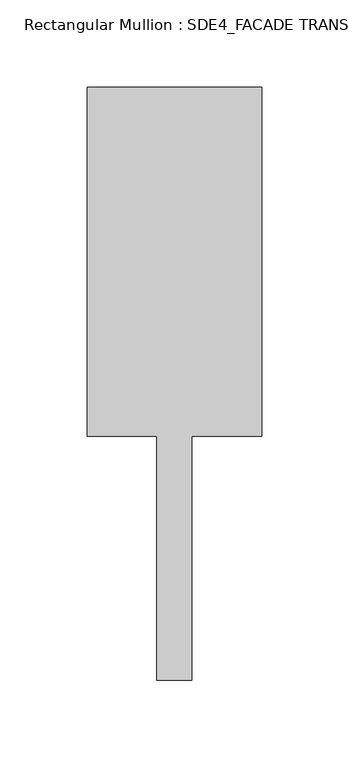
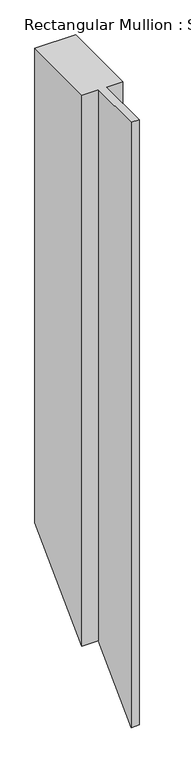
"""IFC4 building model written with IfcOpenShell, lengths in millimetres: member geometry, Rectangular Mullion : SDE4_FACADE TRANSOM TYPE 1."""

from ifc_helpers import new_model, si_unit, origin, place, context, project, spatial, faceted_brep, source, transform, mapped, element, save


def rectangular_mullion_sde4_facade_transom_type_1_05d00b60(model_context):
    return source(origin(), model_context, "Body", "Brep", [
        faceted_brep([(50.0, 132.5, 0.0), (-50.0, 132.5, 0.0), (-50.0, -67.5, 0.0), (-10.0, -67.5, 0.0), (-10.0, -207.5, 0.0), (10.0, -207.5, 0.0), (10.0, -67.5, 0.0), (50.0, -67.5, 0.0), (50.0, 132.5, -1229.9183253), (-50.0, 132.5, -1229.9183253), (-50.0, -67.5, -1429.9183253), (-10.0, -67.5, -1429.9183253), (-10.0, -207.5, -1569.9183253), (10.0, -207.5, -1569.9183253), (10.0, -67.5, -1429.9183253), (50.0, -67.5, -1429.9183253)], [[[0, 1, 2, 3, 4, 5, 6, 7]], [[1, 0, 8, 9]], [[2, 1, 9, 10]], [[3, 2, 10, 11]], [[4, 3, 11, 12]], [[5, 4, 12, 13]], [[6, 5, 13, 14]], [[7, 6, 14, 15]], [[0, 7, 15, 8]], [[8, 15, 14, 13, 12, 11, 10, 9]]]),
    ])


if __name__ == "__main__":
    model = new_model("IFC4")
    model_context = context("Model", 3, world=origin())
    ifc_project = project(units=[si_unit("LENGTHUNIT", "METRE", prefix="MILLI")], contexts=[model_context])
    site = spatial("IfcSite", under=ifc_project)
    building = spatial("IfcBuilding", under=site)
    placement = place(None, origin())
    rectangular_mullion_sde4_facade_transom_type_1_shape = rectangular_mullion_sde4_facade_transom_type_1_05d00b60(model_context)
    element("IfcMember", 1, ObjectType="Rectangular Mullion : SDE4_FACADE TRANSOM TYPE 1", at=placement, inside=building, context=model_context, shape_type="MappedRepresentation", body=[
        mapped(rectangular_mullion_sde4_facade_transom_type_1_shape, transform((0.0, 0.0, 0.0), x_axis=(1.0, 0.0, 0.0), y_axis=(0.0, 1.0, 0.0), z_axis=(0.0, 0.0, 1.0))),
    ])
    save(model, "model.ifc")

# Revit data of these elements
# Type "Rectangular Mullion : SDE4_FACADE TRANSOM TYPE 1"
#   built-in parameter 1007322 = 1.11549 (stored number, unit not read)
#   built-in parameter 1007321 = 0.164042 (stored number, unit not read)
#   built-in parameter 1007320 = 0.164042 (stored number, unit not read)
